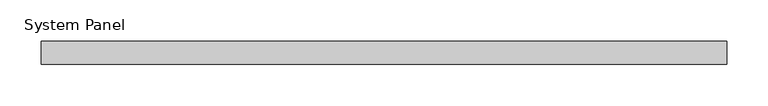
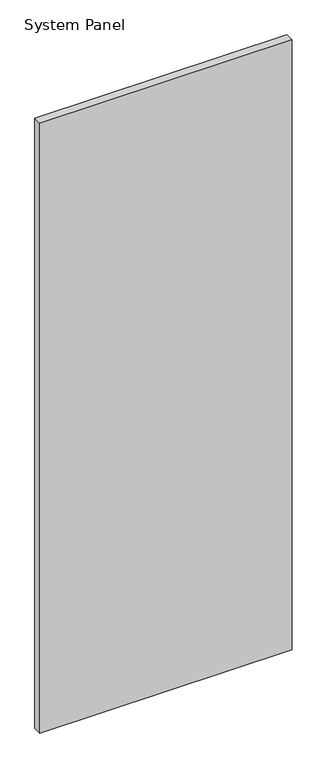
"""IFC4 building model written with IfcOpenShell, lengths in millimetres: plate geometry, System Panel : Schueco_HI_28mm_DoubGlz."""

import ifcopenshell
import ifcopenshell.guid

model = None  # the IFC model being written
_history = None  # IfcOwnerHistory: only IFC2X3 demands one
_inside = {}  # id of a spatial element -> (the spatial element, [elements in it])
_under = {}  # id of a project, library or spatial element -> (it, [spatial elements below it])
_declared = {}  # id of a project -> (the project, [libraries it declares])
_typed = {}  # id of a type object -> (the type object, [elements of that type])
_made_of = {}  # id of a material, layer set ... -> (it, [elements and type objects made of it])


def new_model(schema):
    """Start an empty IFC model of exactly this schema.

    Asked for "IFC4X3", IfcOpenShell would pick the latest addendum, in which some entities
    have other attributes; the version numbers below select the first issue.
    IFC2X3 requires an IfcOwnerHistory on every rooted entity: one is made here for all.
    """
    global model, _history
    if schema == "IFC4X3":
        model = ifcopenshell.file(schema_version=(4, 3, 0, 0))
    else:
        model = ifcopenshell.file(schema=schema)
    _inside.clear()
    _under.clear()
    _declared.clear()
    _typed.clear()
    _made_of.clear()
    _history = None
    if model.schema == "IFC2X3":
        org = make("IfcOrganization", Name="unknown")
        user = make(
            "IfcPersonAndOrganization",
            ThePerson=make("IfcPerson", FamilyName="unknown"),
            TheOrganization=org,
        )
        app = make(
            "IfcApplication",
            ApplicationDeveloper=org,
            Version="unknown",
            ApplicationFullName="unknown",
            ApplicationIdentifier="unknown",
        )
        _history = make(
            "IfcOwnerHistory",
            OwningUser=user,
            OwningApplication=app,
            ChangeAction="ADDED",
            CreationDate=0,
        )
    return model


def make(cls, **values):
    """One entity of the class cls with the attributes given. An attribute that is None is left unset."""
    return model.create_entity(
        cls, **{name: value for name, value in values.items() if value is not None}
    )


def rooted(cls, **values):
    """An entity with a GlobalId (a new one), such as an element, a storey or a relation."""
    return make(cls, GlobalId=ifcopenshell.guid.new(), OwnerHistory=_history, **values)


def si_unit(unit_type, name, prefix=None):
    """IfcSIUnit, for example si_unit("LENGTHUNIT", "METRE", prefix="MILLI")."""
    return make("IfcSIUnit", UnitType=unit_type, Prefix=prefix, Name=name)


def assignment(units):
    """IfcUnitAssignment: the units of a project."""
    return None if units is None else make("IfcUnitAssignment", Units=units)


def point(xyz):
    """IfcCartesianPoint."""
    return None if xyz is None else make("IfcCartesianPoint", Coordinates=xyz)


def direction(xyz):
    """IfcDirection."""
    return None if xyz is None else make("IfcDirection", DirectionRatios=xyz)


def frame(location, z_axis=None, x_axis=None):
    """IfcAxis2Placement3D, a coordinate frame: its origin and axes. An axis left out is left unset."""
    return make(
        "IfcAxis2Placement3D",
        Location=point(location),
        Axis=direction(z_axis),
        RefDirection=direction(x_axis),
    )


def origin():
    """The frame at (0, 0, 0) with its axes left unset."""
    return frame((0.0, 0.0, 0.0))


def origin_with_axes():
    """The frame at (0, 0, 0) with the z axis (0, 0, 1) and the x axis (1, 0, 0) written out."""
    return frame((0.0, 0.0, 0.0), z_axis=(0.0, 0.0, 1.0), x_axis=(1.0, 0.0, 0.0))


def place(relative_to, where):
    """IfcLocalPlacement: puts the frame where relative to a parent placement (None: the world)."""
    return make(
        "IfcLocalPlacement", PlacementRelTo=relative_to, RelativePlacement=where
    )


def context(
    kind, dimensions, precision=None, world=None, true_north=None, identifier=None
):
    """IfcGeometricRepresentationContext, for example the 3D "Model" context."""
    return make(
        "IfcGeometricRepresentationContext",
        ContextIdentifier=identifier,
        ContextType=kind,
        CoordinateSpaceDimension=dimensions,
        Precision=precision,
        WorldCoordinateSystem=world,
        TrueNorth=true_north,
    )


def project(units=None, contexts=None):
    """IfcProject with its units and contexts."""
    return rooted(
        "IfcProject",
        Name="project",
        RepresentationContexts=contexts,
        UnitsInContext=assignment(units),
    )


def spatial(cls, under=None, at=None, **own):
    """A site, building, storey or space (cls), placed at a placement, below another one or the project."""
    s = rooted(cls, ObjectPlacement=at, **own)
    if under is not None:
        _under.setdefault(under.id(), (under, []))[1].append(s)
    return s


def polyline(points):
    """IfcPolyline through the points."""
    return make("IfcPolyline", Points=[point(p) for p in points])


def outline(outer, holes=None, kind="AREA"):
    """IfcArbitraryClosedProfileDef: a profile drawn as a closed curve; with holes, ...WithVoids."""
    if holes is None:
        return make("IfcArbitraryClosedProfileDef", ProfileType=kind, OuterCurve=outer)
    return make(
        "IfcArbitraryProfileDefWithVoids",
        ProfileType=kind,
        OuterCurve=outer,
        InnerCurves=holes,
    )


def extrude(swept, where, along, depth):
    """IfcExtrudedAreaSolid: the profile swept, set in the frame where, extruded along a direction by depth."""
    return make(
        "IfcExtrudedAreaSolid",
        SweptArea=swept,
        Position=where,
        ExtrudedDirection=direction(along),
        Depth=depth,
    )


def shape(context_of_items, identifier, shape_type, items):
    """IfcShapeRepresentation: the items that make up one representation, for example the "Body"."""
    return make(
        "IfcShapeRepresentation",
        ContextOfItems=context_of_items,
        RepresentationIdentifier=identifier,
        RepresentationType=shape_type,
        Items=items,
    )


def source(mapping_origin, context_of_items, identifier, shape_type, items):
    """IfcRepresentationMap: a shape defined once, which mapped items show again and again."""
    return make(
        "IfcRepresentationMap",
        MappingOrigin=mapping_origin,
        MappedRepresentation=shape(context_of_items, identifier, shape_type, items),
    )


def transform(
    local_origin,
    x_axis=None,
    y_axis=None,
    z_axis=None,
    scale=None,
    scale2=None,
    scale3=None,
    uniform=True,
):
    """IfcCartesianTransformationOperator3D, or its non-uniform kind. x_axis, y_axis, z_axis: its Axis1, 2, 3."""
    if uniform:
        return make(
            "IfcCartesianTransformationOperator3D",
            Axis1=direction(x_axis),
            Axis2=direction(y_axis),
            LocalOrigin=point(local_origin),
            Scale=scale,
            Axis3=direction(z_axis),
        )
    return make(
        "IfcCartesianTransformationOperator3DnonUniform",
        Axis1=direction(x_axis),
        Axis2=direction(y_axis),
        LocalOrigin=point(local_origin),
        Scale=scale,
        Axis3=direction(z_axis),
        Scale2=scale2,
        Scale3=scale3,
    )


def mapped(mapping_source, mapping_target):
    """IfcMappedItem: shows the shape of a source again, moved by a transform."""
    return make(
        "IfcMappedItem", MappingSource=mapping_source, MappingTarget=mapping_target
    )


def made_of(thing, what):
    """Note that an element or type object is made of a material, layer set ...; save() writes the relation."""
    if what is not None:
        _made_of.setdefault(what.id(), (what, []))[1].append(thing)
    return thing


def element(
    cls,
    number,
    at=None,
    inside=None,
    cuts=None,
    type_object=None,
    material=None,
    context=None,
    identifier="Body",
    shape_type=None,
    held_by="IfcProductDefinitionShape",
    body=None,
    shapes=None,
    **own,
):
    """One element of the class cls, such as IfcWall. Its Tag is "e" and its number.

    at: its placement. inside: the storey or other place that contains it. cuts: it is an
    opening in that element (IfcRelVoidsElement). A single representation is given by context,
    identifier, shape_type and body (its items); several are given by shapes. held_by: the class
    of the entity that holds the representations. save() writes the other relations.
    """
    e = rooted(cls, Tag="e%d" % number, ObjectPlacement=at, **own)
    if body is not None:
        shapes = [shape(context, identifier, shape_type, body)]
    if shapes is not None:
        e.Representation = make(held_by, Representations=shapes)
    if inside is not None:
        _inside.setdefault(inside.id(), (inside, []))[1].append(e)
    if cuts is not None:
        rooted(
            "IfcRelVoidsElement", RelatingBuildingElement=cuts, RelatedOpeningElement=e
        )
    if type_object is not None:
        _typed.setdefault(type_object.id(), (type_object, []))[1].append(e)
    return made_of(e, material)


def aggregate(whole, parts):
    """IfcRelAggregates: a whole, such as a stair, and the parts it consists of."""
    return rooted("IfcRelAggregates", RelatingObject=whole, RelatedObjects=parts)


def save(model, path):
    """Write the relations noted so far, then the file.

    IfcRelAggregates (storeys below a building ...), IfcRelContainedInSpatialStructure (elements
    in a storey), IfcRelDefinesByType, IfcRelAssociatesMaterial and IfcRelDeclares: one each for
    every whole, place, type object, material and project.
    """
    for whole, parts in _under.values():
        aggregate(whole, parts)
    for where, things in _inside.values():
        rooted(
            "IfcRelContainedInSpatialStructure",
            RelatedElements=things,
            RelatingStructure=where,
        )
    for kind, things in _typed.values():
        rooted("IfcRelDefinesByType", RelatedObjects=things, RelatingType=kind)
    for what, things in _made_of.values():
        rooted("IfcRelAssociatesMaterial", RelatedObjects=things, RelatingMaterial=what)
    for by, libraries in _declared.values():
        rooted("IfcRelDeclares", RelatingContext=by, RelatedDefinitions=libraries)
    model.write(path)


def system_panel_b62043d7(model_context):
    return source(origin(), model_context, "Body", "SweptSolid", [
        extrude(outline(polyline([(416.5, -28.0), (-416.5, -28.0), (-416.5, 0.0), (416.5, 0.0), (416.5, -28.0)])), origin_with_axes(), (0.0, 0.0, 1.0), 2128.0),
    ])


if __name__ == "__main__":
    model = new_model("IFC4")
    model_context = context("Model", 3, world=origin())
    ifc_project = project(units=[si_unit("LENGTHUNIT", "METRE", prefix="MILLI")], contexts=[model_context])
    site = spatial("IfcSite", under=ifc_project)
    building = spatial("IfcBuilding", under=site)
    placement = place(None, origin())
    system_panel_shape = system_panel_b62043d7(model_context)
    element("IfcPlate", 1, ObjectType="System Panel : Schueco_HI_28mm_DoubGlz", at=placement, inside=building, context=model_context, shape_type="MappedRepresentation", body=[
        mapped(system_panel_shape, transform((0.0, 0.0, 0.0), x_axis=(1.0, 0.0, 0.0), y_axis=(0.0, 1.0, 0.0), z_axis=(0.0, 0.0, 1.0))),
    ])
    save(model, "model.ifc")

# Revit data of these elements
# Type "System Panel : Schueco_HI_28mm_DoubGlz"
#   Model = "Double glazing 28mm"
# Element 1 (IfcPlate, "System Panel : Schueco_HI_28mm_DoubGlz")
#   Materials on its faces: "Glass"
# Materials
#   "Glass": class "Glass", colour RGB 128 128 255, transparency 0.75, Description = "Soda Lime Glass", Cost = 0
